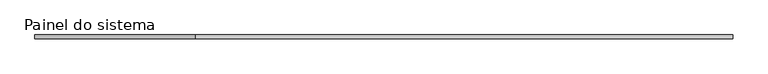
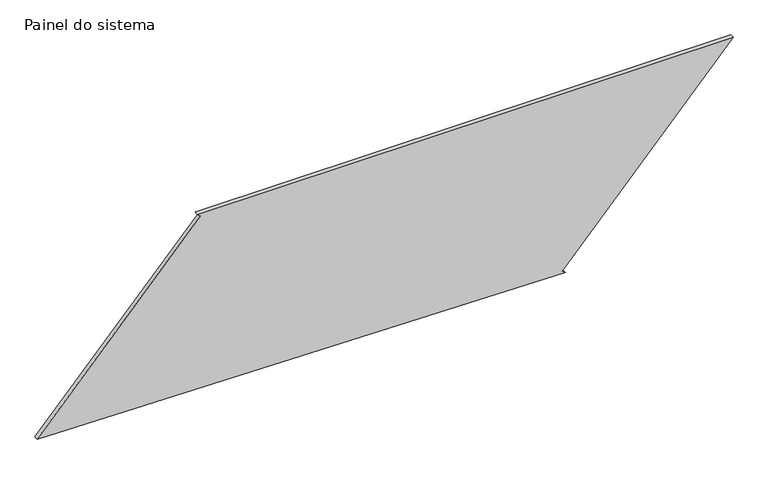
"""IFC4 building model written with IfcOpenShell, lengths in millimetres: plate geometry, Painel do sistema : Envidraçado."""

import ifcopenshell
import ifcopenshell.guid

model = None  # the IFC model being written
_history = None  # IfcOwnerHistory: only IFC2X3 demands one
_inside = {}  # id of a spatial element -> (the spatial element, [elements in it])
_under = {}  # id of a project, library or spatial element -> (it, [spatial elements below it])
_declared = {}  # id of a project -> (the project, [libraries it declares])
_typed = {}  # id of a type object -> (the type object, [elements of that type])
_made_of = {}  # id of a material, layer set ... -> (it, [elements and type objects made of it])


def new_model(schema):
    """Start an empty IFC model of exactly this schema.

    Asked for "IFC4X3", IfcOpenShell would pick the latest addendum, in which some entities
    have other attributes; the version numbers below select the first issue.
    IFC2X3 requires an IfcOwnerHistory on every rooted entity: one is made here for all.
    """
    global model, _history
    if schema == "IFC4X3":
        model = ifcopenshell.file(schema_version=(4, 3, 0, 0))
    else:
        model = ifcopenshell.file(schema=schema)
    _inside.clear()
    _under.clear()
    _declared.clear()
    _typed.clear()
    _made_of.clear()
    _history = None
    if model.schema == "IFC2X3":
        org = make("IfcOrganization", Name="unknown")
        user = make(
            "IfcPersonAndOrganization",
            ThePerson=make("IfcPerson", FamilyName="unknown"),
            TheOrganization=org,
        )
        app = make(
            "IfcApplication",
            ApplicationDeveloper=org,
            Version="unknown",
            ApplicationFullName="unknown",
            ApplicationIdentifier="unknown",
        )
        _history = make(
            "IfcOwnerHistory",
            OwningUser=user,
            OwningApplication=app,
            ChangeAction="ADDED",
            CreationDate=0,
        )
    return model


def make(cls, **values):
    """One entity of the class cls with the attributes given. An attribute that is None is left unset."""
    return model.create_entity(
        cls, **{name: value for name, value in values.items() if value is not None}
    )


def rooted(cls, **values):
    """An entity with a GlobalId (a new one), such as an element, a storey or a relation."""
    return make(cls, GlobalId=ifcopenshell.guid.new(), OwnerHistory=_history, **values)


def si_unit(unit_type, name, prefix=None):
    """IfcSIUnit, for example si_unit("LENGTHUNIT", "METRE", prefix="MILLI")."""
    return make("IfcSIUnit", UnitType=unit_type, Prefix=prefix, Name=name)


def assignment(units):
    """IfcUnitAssignment: the units of a project."""
    return None if units is None else make("IfcUnitAssignment", Units=units)


def point(xyz):
    """IfcCartesianPoint."""
    return None if xyz is None else make("IfcCartesianPoint", Coordinates=xyz)


def direction(xyz):
    """IfcDirection."""
    return None if xyz is None else make("IfcDirection", DirectionRatios=xyz)


def frame(location, z_axis=None, x_axis=None):
    """IfcAxis2Placement3D, a coordinate frame: its origin and axes. An axis left out is left unset."""
    return make(
        "IfcAxis2Placement3D",
        Location=point(location),
        Axis=direction(z_axis),
        RefDirection=direction(x_axis),
    )


def origin():
    """The frame at (0, 0, 0) with its axes left unset."""
    return frame((0.0, 0.0, 0.0))


def place(relative_to, where):
    """IfcLocalPlacement: puts the frame where relative to a parent placement (None: the world)."""
    return make(
        "IfcLocalPlacement", PlacementRelTo=relative_to, RelativePlacement=where
    )


def context(
    kind, dimensions, precision=None, world=None, true_north=None, identifier=None
):
    """IfcGeometricRepresentationContext, for example the 3D "Model" context."""
    return make(
        "IfcGeometricRepresentationContext",
        ContextIdentifier=identifier,
        ContextType=kind,
        CoordinateSpaceDimension=dimensions,
        Precision=precision,
        WorldCoordinateSystem=world,
        TrueNorth=true_north,
    )


def project(units=None, contexts=None):
    """IfcProject with its units and contexts."""
    return rooted(
        "IfcProject",
        Name="project",
        RepresentationContexts=contexts,
        UnitsInContext=assignment(units),
    )


def spatial(cls, under=None, at=None, **own):
    """A site, building, storey or space (cls), placed at a placement, below another one or the project."""
    s = rooted(cls, ObjectPlacement=at, **own)
    if under is not None:
        _under.setdefault(under.id(), (under, []))[1].append(s)
    return s


def polyline(points):
    """IfcPolyline through the points."""
    return make("IfcPolyline", Points=[point(p) for p in points])


def outline(outer, holes=None, kind="AREA"):
    """IfcArbitraryClosedProfileDef: a profile drawn as a closed curve; with holes, ...WithVoids."""
    if holes is None:
        return make("IfcArbitraryClosedProfileDef", ProfileType=kind, OuterCurve=outer)
    return make(
        "IfcArbitraryProfileDefWithVoids",
        ProfileType=kind,
        OuterCurve=outer,
        InnerCurves=holes,
    )


def extrude(swept, where, along, depth):
    """IfcExtrudedAreaSolid: the profile swept, set in the frame where, extruded along a direction by depth."""
    return make(
        "IfcExtrudedAreaSolid",
        SweptArea=swept,
        Position=where,
        ExtrudedDirection=direction(along),
        Depth=depth,
    )


def shape(context_of_items, identifier, shape_type, items):
    """IfcShapeRepresentation: the items that make up one representation, for example the "Body"."""
    return make(
        "IfcShapeRepresentation",
        ContextOfItems=context_of_items,
        RepresentationIdentifier=identifier,
        RepresentationType=shape_type,
        Items=items,
    )


def source(mapping_origin, context_of_items, identifier, shape_type, items):
    """IfcRepresentationMap: a shape defined once, which mapped items show again and again."""
    return make(
        "IfcRepresentationMap",
        MappingOrigin=mapping_origin,
        MappedRepresentation=shape(context_of_items, identifier, shape_type, items),
    )


def transform(
    local_origin,
    x_axis=None,
    y_axis=None,
    z_axis=None,
    scale=None,
    scale2=None,
    scale3=None,
    uniform=True,
):
    """IfcCartesianTransformationOperator3D, or its non-uniform kind. x_axis, y_axis, z_axis: its Axis1, 2, 3."""
    if uniform:
        return make(
            "IfcCartesianTransformationOperator3D",
            Axis1=direction(x_axis),
            Axis2=direction(y_axis),
            LocalOrigin=point(local_origin),
            Scale=scale,
            Axis3=direction(z_axis),
        )
    return make(
        "IfcCartesianTransformationOperator3DnonUniform",
        Axis1=direction(x_axis),
        Axis2=direction(y_axis),
        LocalOrigin=point(local_origin),
        Scale=scale,
        Axis3=direction(z_axis),
        Scale2=scale2,
        Scale3=scale3,
    )


def mapped(mapping_source, mapping_target):
    """IfcMappedItem: shows the shape of a source again, moved by a transform."""
    return make(
        "IfcMappedItem", MappingSource=mapping_source, MappingTarget=mapping_target
    )


def made_of(thing, what):
    """Note that an element or type object is made of a material, layer set ...; save() writes the relation."""
    if what is not None:
        _made_of.setdefault(what.id(), (what, []))[1].append(thing)
    return thing


def element(
    cls,
    number,
    at=None,
    inside=None,
    cuts=None,
    type_object=None,
    material=None,
    context=None,
    identifier="Body",
    shape_type=None,
    held_by="IfcProductDefinitionShape",
    body=None,
    shapes=None,
    **own,
):
    """One element of the class cls, such as IfcWall. Its Tag is "e" and its number.

    at: its placement. inside: the storey or other place that contains it. cuts: it is an
    opening in that element (IfcRelVoidsElement). A single representation is given by context,
    identifier, shape_type and body (its items); several are given by shapes. held_by: the class
    of the entity that holds the representations. save() writes the other relations.
    """
    e = rooted(cls, Tag="e%d" % number, ObjectPlacement=at, **own)
    if body is not None:
        shapes = [shape(context, identifier, shape_type, body)]
    if shapes is not None:
        e.Representation = make(held_by, Representations=shapes)
    if inside is not None:
        _inside.setdefault(inside.id(), (inside, []))[1].append(e)
    if cuts is not None:
        rooted(
            "IfcRelVoidsElement", RelatingBuildingElement=cuts, RelatedOpeningElement=e
        )
    if type_object is not None:
        _typed.setdefault(type_object.id(), (type_object, []))[1].append(e)
    return made_of(e, material)


def aggregate(whole, parts):
    """IfcRelAggregates: a whole, such as a stair, and the parts it consists of."""
    return rooted("IfcRelAggregates", RelatingObject=whole, RelatedObjects=parts)


def save(model, path):
    """Write the relations noted so far, then the file.

    IfcRelAggregates (storeys below a building ...), IfcRelContainedInSpatialStructure (elements
    in a storey), IfcRelDefinesByType, IfcRelAssociatesMaterial and IfcRelDeclares: one each for
    every whole, place, type object, material and project.
    """
    for whole, parts in _under.values():
        aggregate(whole, parts)
    for where, things in _inside.values():
        rooted(
            "IfcRelContainedInSpatialStructure",
            RelatedElements=things,
            RelatingStructure=where,
        )
    for kind, things in _typed.values():
        rooted("IfcRelDefinesByType", RelatedObjects=things, RelatingType=kind)
    for what, things in _made_of.values():
        rooted("IfcRelAssociatesMaterial", RelatedObjects=things, RelatingMaterial=what)
    for by, libraries in _declared.values():
        rooted("IfcRelDeclares", RelatingContext=by, RelatedDefinitions=libraries)
    model.write(path)


def painel_do_sistema_fba78f14(model_context):
    return source(origin(), model_context, "Body", "SweptSolid", [
        extrude(outline(polyline([(0.0, 1157.8929446), (16.8339598, 1139.4100391), (1223.5447416, 2238.464556), (1223.5447416, -1207.461375), (1206.7107818, -1188.9784695), (54.4238329, -2238.464556), (0.0, 1157.8929446)])), frame((0.0, 24.5, 0.0), z_axis=(0.0, 1.0, 0.0), x_axis=(0.0, 0.0, 1.0)), (0.0, 0.0, 1.0), 25.0),
    ])


if __name__ == "__main__":
    model = new_model("IFC4")
    model_context = context("Model", 3, world=origin())
    ifc_project = project(units=[si_unit("LENGTHUNIT", "METRE", prefix="MILLI")], contexts=[model_context])
    site = spatial("IfcSite", under=ifc_project)
    building = spatial("IfcBuilding", under=site)
    placement = place(None, origin())
    painel_do_sistema_shape = painel_do_sistema_fba78f14(model_context)
    element("IfcPlate", 1, ObjectType="Painel do sistema : Envidraçado", at=placement, inside=building, context=model_context, shape_type="MappedRepresentation", body=[
        mapped(painel_do_sistema_shape, transform((0.0, 0.0, 0.0), x_axis=(1.0, 0.0, 0.0), y_axis=(0.0, 1.0, 0.0), z_axis=(0.0, 0.0, 1.0))),
    ])
    save(model, "model.ifc")

# Revit data of these elements
# Type "Painel do sistema : Envidraçado"
#   Construction Type Id = "GSP4R"
#   Analytic Construction = "Vidraça única Pilkington 1/8 pol"
#   Visual Light Transmittance = 0.9
#   Solar Heat Gain Coefficient = 0.86
#   Heat Transfer Coefficient (U) = 6.7069 W/(m²·K)
# Element 1 (IfcPlate, "Painel do sistema : Envidraçado")
#   Materials on its faces: "Vidro"
# Materials
#   "Vidro": class "Vidro", colour RGB 0 128 192, transparency 0.9, Description = "Vidro de sílica", Cost = 0
